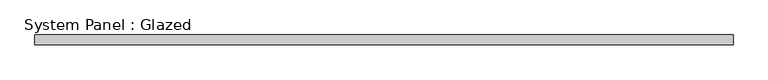
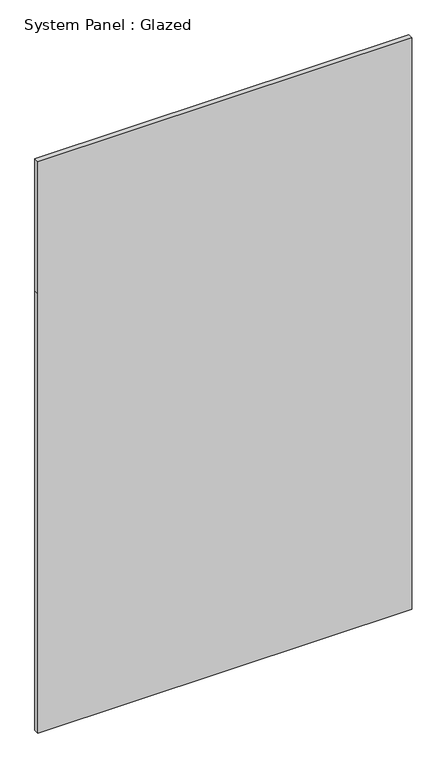
"""IFC4 building model written with IfcOpenShell, lengths in millimetres: plate geometry, System Panel : Glazed."""

from ifc_helpers import new_model, si_unit, frame, origin, place, context, project, spatial, polyline, outline, extrude, source, transform, mapped, element, save


def system_panel_glazed_640a10fc(model_context):
    return source(origin(), model_context, "Body", "SweptSolid", [
        extrude(outline(polyline([(0.0, -905.5833335), (0.0, 905.5833335), (2250.0, 905.5833335), (2925.0, 905.5833335), (2925.0, -905.5833335), (2250.0, -905.5833335), (0.0, -905.5833335)])), frame((0.0, 24.5, 0.0), z_axis=(0.0, 1.0, 0.0), x_axis=(0.0, 0.0, 1.0)), (0.0, 0.0, 1.0), 25.0),
    ])


if __name__ == "__main__":
    model = new_model("IFC4")
    model_context = context("Model", 3, world=origin())
    ifc_project = project(units=[si_unit("LENGTHUNIT", "METRE", prefix="MILLI")], contexts=[model_context])
    site = spatial("IfcSite", under=ifc_project)
    building = spatial("IfcBuilding", under=site)
    placement = place(None, origin())
    system_panel_glazed_shape = system_panel_glazed_640a10fc(model_context)
    element("IfcPlate", 1, ObjectType="System Panel : Glazed", at=placement, inside=building, context=model_context, shape_type="MappedRepresentation", body=[
        mapped(system_panel_glazed_shape, transform((0.0, 0.0, 0.0), x_axis=(1.0, 0.0, 0.0), y_axis=(0.0, 1.0, 0.0), z_axis=(0.0, 0.0, 1.0))),
    ])
    save(model, "model.ifc")

# Revit data of these elements
# Element 1 (IfcPlate, "System Panel : Glazed")
#   Materials on its faces: "Glass"
# Materials
#   "Glass": class "Glass", colour RGB 0 128 192, transparency 0.9
